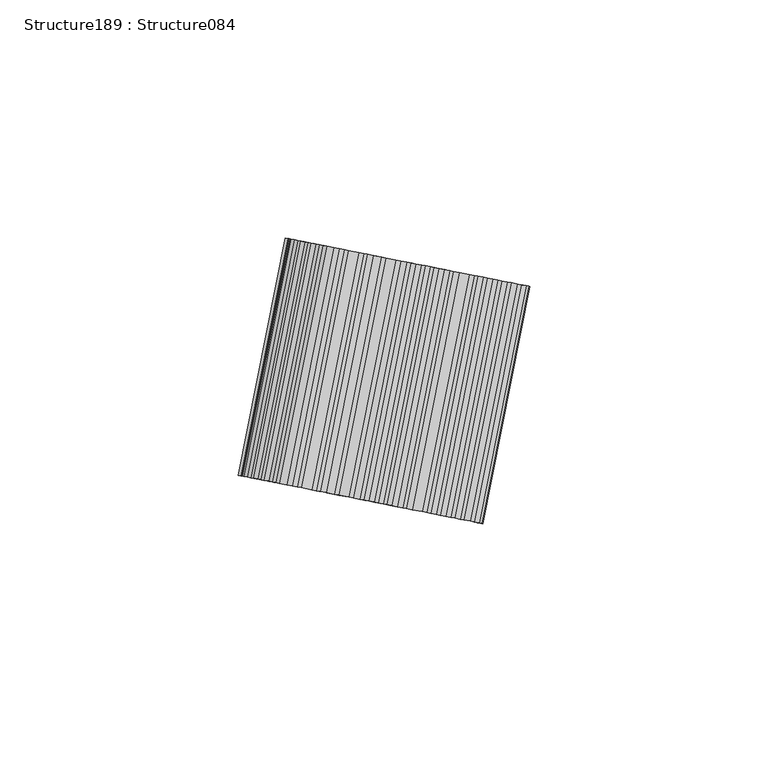
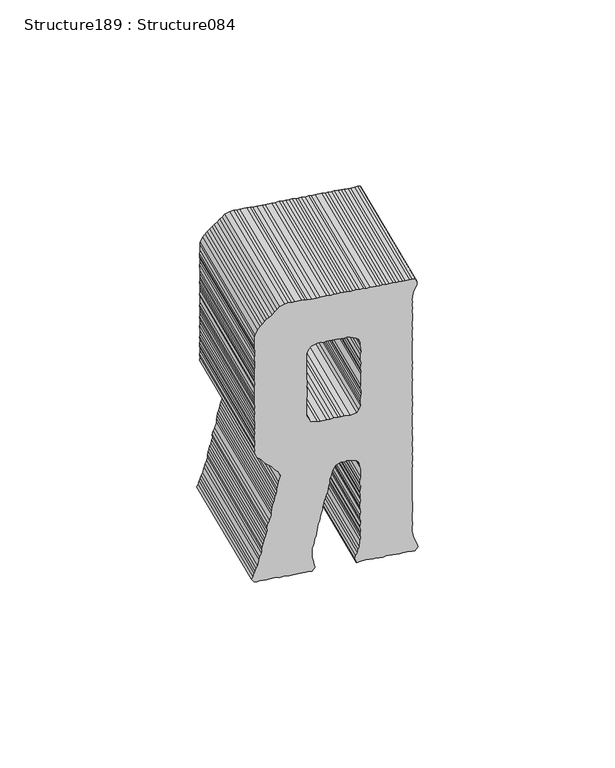
"""IFC4 building model written with IfcOpenShell, lengths in millimetres: proxy geometry, Structure189 : Structure084."""

from ifc_helpers import new_model, si_unit, frame, origin, place, context, project, spatial, polyline, outline, extrude, source, transform, mapped, element, save


def structure189_structure084_a6cd63ed(model_context):
    return source(origin(), model_context, "Body", "SweptSolid", [
        extrude(outline(polyline([(0.7877723, 0.0), (1.9464015, -0.1991228), (2.8602744, -0.225849), (4.1191818, -0.5725383), (5.014805, -0.7264607), (5.8881786, -1.0119464), (7.2131992, -0.9739456), (7.9618749, -1.2329462), (10.1385127, -1.6070246), (11.3090794, -1.6778664), (12.311293, -1.9804401), (13.2111243, -2.1350857), (14.2117928, -2.4424483), (15.4109212, -2.3828117), (16.5195828, -2.8390667), (17.4342994, -2.8608834), (18.6150357, -2.933473), (20.3591199, -3.4989322), (21.6394332, -3.7189677), (22.5801144, -3.6149141), (23.6845679, -4.0704459), (24.6308598, -3.9673566), (25.7800208, -4.1648522), (26.5039924, -4.5549941), (27.5279624, -4.7309743), (28.8526323, -4.6929133), (29.8357525, -5.1275927), (30.776083, -5.0234788), (32.5416935, -6.2493551), (32.9031424, -7.2342724), (33.5574941, -8.0085018), (34.477038, -8.823614), (35.0861234, -9.8507291), (35.972525, -11.5876372), (36.8685591, -12.5290416), (37.5229108, -13.303271), (37.9287766, -14.029741), (39.5076035, -14.8278254), (41.6445256, -14.6683321), (42.9644943, -14.6345176), (43.9051754, -14.530464), (45.0599472, -14.7289238), (46.0220341, -14.4982164), (46.9627152, -14.3941628), (48.1392433, -14.4660291), (49.0957798, -14.2340066), (50.041228, -14.1358267), (51.0844997, -14.1847914), (52.1563332, -14.1032778), (53.4327891, -14.3226503), (55.3194114, -14.1154471), (56.4288566, -13.779371), (57.6236345, -13.7240411), (58.7537019, -14.0536423), (59.5858309, -13.7955458), (60.7623591, -13.8674121), (61.6189076, -13.4882341), (62.7924221, -13.5545279), (63.7358265, -13.4556357), (64.9285003, -13.3999442), (65.8244741, -13.5539269), (66.898061, -13.4727145), (68.1350915, -13.1589264), (69.328609, -13.0983255), (71.318233, -13.0438502), (72.1765349, -12.6649735), (73.2419139, -12.587405), (74.0793029, -12.3302124), (75.2758945, -12.2748331), (76.003044, -11.8734165), (76.8931166, -12.8137963), (76.8480367, -13.8638733), (76.5842472, -14.6110041), (76.5400111, -15.6561716), (76.3416115, -16.8105927), (76.0343091, -17.8109106), (75.7045271, -19.7298024), (75.8093424, -20.6702534), (75.3295446, -21.9117003), (75.2811608, -23.7435663), (74.9337097, -25.0027039), (74.4272846, -27.9494232), (74.4005969, -28.8672741), (73.987756, -29.7191213), (74.0707545, -30.7865166), (72.6138584, -31.5939579), (71.7839977, -31.0552851), (70.7821347, -30.7527716), (69.6713689, -30.2961549), (68.9473974, -29.906013), (66.901912, -29.5544745), (65.7471403, -29.3560146), (64.7624532, -29.718225), (63.8447229, -29.6908359), (62.6738055, -29.6199339), (61.6840006, -29.9762104), (60.4904228, -30.0371621), (59.445047, -29.9878357), (58.3961644, -29.9379067), (57.3516982, -29.8937911), (56.362244, -30.2501279), (55.1913266, -30.1792259), (54.145107, -30.1348089), (53.0523006, -30.3383574), (52.1175809, -30.4434355), (51.2156457, -30.2884283), (50.0229718, -30.3441199), (48.9553464, -30.4263568), (47.8617565, -30.6344641), (47.0534221, -30.7562085), (45.832477, -30.9427894), (44.914396, -30.91534), (43.7173718, -30.9753383), (42.7766906, -31.079392), (41.494624, -30.8590552), (40.6854459, -30.985709), (39.5926997, -31.1889068), (38.2679695, -31.2273185), (36.4472301, -31.8368424), (35.5455414, -33.2664481), (35.3262292, -34.5425532), (34.9408158, -35.2684206), (34.9738469, -36.5929481), (35.1774557, -38.4731762), (35.8364483, -39.2435098), (37.3094464, -39.8927126), (38.4142507, -40.3483048), (41.3574633, -40.8541273), (42.4292967, -40.7726135), (43.70961, -40.9926491), (44.6888727, -41.4266656), (45.7377553, -41.4765946), (46.525177, -41.4765343), (47.5244428, -41.783656), (48.8103669, -42.0046557), (49.6810775, -42.2846293), (50.8784525, -42.2246912), (51.9076827, -42.4015754), (52.649904, -42.6645212), (53.6552737, -42.9676373), (54.9802942, -42.9296365), (56.0035629, -43.1054961), (56.8555307, -43.5176357), (57.7515045, -43.6716184), (58.9488796, -43.6116803), (60.0554372, -44.0675738), (61.0990597, -44.1165988), (61.869492, -44.2490058), (63.0007539, -44.5737579), (63.9372269, -44.468981), (66.2885299, -44.6124122), (67.125919, -44.3552198), (68.4493124, -44.3266872), (69.3028472, -43.9419368), (70.5019756, -43.8823), (71.6935756, -44.6185287), (71.3461245, -45.8776663), (70.9132807, -46.8564085), (70.759298, -47.7523823), (70.7307966, -48.6702824), (70.6639602, -49.846953), (70.3566579, -50.8472709), (70.3341179, -51.7661955), (70.1575351, -52.7936724), (69.7472914, -53.6409116), (69.69625, -54.689964), (69.3228948, -56.8623937), (69.2778149, -57.9124707), (68.992269, -58.786195), (68.6181303, -60.9631834), (68.5955903, -61.8821081), (68.4416077, -62.7780818), (67.1345464, -63.4762479), (66.0458878, -62.8930979), (65.1969939, -62.4861801), (64.1318451, -61.7767379), (63.4057694, -61.3862343), (61.4454907, -60.5179), (60.4218712, -60.3419801), (58.3267691, -60.2476341), (57.4807627, -59.8365192), (56.1757452, -59.7476251), (55.2985141, -59.4614765), (54.2305381, -59.5436531), (51.2834681, -59.0371677), (50.3063094, -58.6035128), (49.28269, -58.4275929), (47.9738151, -58.3380358), (46.0598327, -58.0090975), (45.0553067, -57.7010719), (44.0334407, -57.5254533), (42.9872211, -57.4810364), (39.0186357, -56.7989926), (37.9732599, -56.7496663), (36.9678903, -56.4465501), (35.6637165, -56.3527466), (34.6422011, -56.1771882), (33.8931746, -55.9181274), (32.8499028, -55.8691626), (31.5636281, -55.6481026), (30.5617652, -55.3455891), (29.6714021, -55.1925707), (28.7480611, -55.1642173), (27.5989002, -54.9667218), (26.7434256, -54.5539796), (25.5695604, -54.4876254), (24.5262885, -54.4386606), (23.4214843, -53.9830685), (22.6245944, -53.9815015), (21.6235752, -53.6740786), (20.3206618, -53.5855461), (19.2756365, -53.53628), (18.5509637, -53.1460175), (17.268897, -52.9256807), (16.4593683, -53.0522743), (15.300739, -52.8531514), (14.4321325, -52.5735395), (13.3871074, -52.5242734), (12.1225891, -52.1766198), (11.3803678, -51.9136741), (10.2086067, -51.8476815), (8.0263581, -51.4726388), (7.2362735, -51.4671869), (6.1085182, -51.1430375), (5.2354954, -50.8576121), (4.0800223, -50.6590317), (3.1400425, -50.7632059), (2.0122874, -50.4390565), (1.0892969, -50.4107634), (-0.1431529, -49.933234), (-1.1706297, -49.7566511), (-2.2147453, -49.7125958), (-2.9573172, -49.4495898), (-4.0087969, -49.4042689), (-5.0080628, -49.0971473), (-6.2887267, -48.8770515), (-7.1035156, -49.0027411), (-8.3620724, -48.656112), (-9.1102552, -48.3921417), (-10.1314198, -48.2166437), (-11.1997466, -48.29876), (-12.2051163, -47.9956439), (-13.4854295, -47.7756083), (-14.2776182, -47.7697949), (-16.3227529, -47.4183167), (-17.4331681, -46.9617603), (-18.4993908, -47.0442382), (-19.6267952, -46.7201491), (-20.6781325, -46.6697982), (-21.5523499, -46.3892219), (-23.7729936, -46.2733003), (-24.8401259, -46.3505675), (-25.6975181, -46.734655), (-26.7864672, -46.9388664), (-27.9612419, -46.8673015), (-28.903386, -46.1836924), (-28.8523447, -45.1346399), (-28.6983018, -44.2383154), (-28.3526042, -42.9788764), (-28.220378, -42.2094962), (-28.1483637, -41.0384089), (-27.8679957, -40.1591014), (-27.8177379, -39.1146076), (-27.6201821, -37.965096), (-27.3406578, -37.0906979), (-27.2677998, -35.9147012), (-27.010032, -35.1668965), (-26.9597742, -34.1224029), (-26.6073919, -32.072008), (-26.2616943, -30.8125691), (-26.3826552, -29.9996759), (-25.9319123, -28.8936772), (-25.9875436, -27.7006527), (-25.6832549, -26.6947624), (-25.4254871, -25.9469578), (-25.5028748, -24.8805269), (-25.2212466, -24.0064903), (-25.1513363, -22.8350415), (-24.8470476, -21.8291512), (-24.8207105, -20.9112402), (-24.3473674, -19.6737385), (-24.2963261, -18.624686), (-23.8191857, -16.6004256), (-23.6434466, -15.5778582), (-23.3571774, -13.9121535), (-23.1370214, -12.6311389), (-23.1311203, -11.8447418), (-23.0821829, -10.7953277), (-22.707984, -8.6179885), (-22.4263557, -7.743952), (-22.3782019, -6.6990967), (-21.9266152, -5.5881886), (-21.1449177, -4.1383221), (-20.1224106, -3.5266396), (-19.3473977, -2.8677292), (-18.3143703, -2.2578546), (-17.5002006, -1.3395928), (-16.8785896, -0.7897057), (-16.003649, -0.2783015), (-15.0749656, 0.4848928), (-14.3537777, 0.8873339), (-13.1940143, 1.480482), (-11.3979792, 1.9588644), (-10.4794051, 1.9363847), (-8.428309, 1.583882), (-7.1300967, 1.491103), (-6.3554563, 1.3579727), (-5.3765442, 0.9240165), (-4.3546782, 0.7483979), (-3.2867022, 0.8305746), (-1.0232687, 0.1758597), (0.0, 0.0), (0.7877723, 0.0)]), holes=[polyline([(18.9318372, -31.7250019), (19.2826525, -30.471497), (19.2842194, -29.674607), (19.5035317, -28.3985018), (19.9610799, -27.2886183), (20.0100172, -26.2392042), (20.4892615, -24.2153054), (20.3840956, -23.2747941), (20.4678464, -21.3085648), (19.6312408, -20.7734262), (18.3769139, -19.6354193), (17.4595343, -19.6080905), (16.1792211, -19.388055), (15.4301946, -19.1289941), (14.2771763, -18.9308356), (13.3629527, -18.9040492), (12.3417881, -18.7285511), (11.0337568, -18.6340846), (8.9865181, -18.2822448), (7.9811484, -17.9791286), (7.0630675, -17.9516793), (6.1670937, -17.7976966), (5.0614456, -17.3470139), (4.1654718, -17.1930312), (2.9889437, -17.1211649), (2.0926191, -16.967122), (1.0925096, -16.6649099), (-0.0840186, -16.5930436), (-0.9582359, -16.3124674), (-2.1130076, -16.1140075), (-3.0310886, -16.0865581), (-3.8996951, -15.8069462), (-5.5492761, -16.1852202), (-6.4511511, -16.8176346), (-7.5496121, -18.6044208), (-7.7253512, -19.6269882), (-7.6009438, -20.4408347), (-8.0334371, -21.4196372), (-8.5841586, -24.6241024), (-8.6784224, -25.9267529), (-8.6799072, -26.7189635), (-9.1123403, -27.6974153), (-9.0314457, -28.7644489), (-8.7006845, -30.671584), (-8.3169861, -31.524938), (-6.8689006, -32.3001919), (-5.9732774, -32.4541143), (-3.7094934, -33.1088896), (-2.7730203, -33.0041127), (-0.5967332, -33.3781309), (0.1279397, -33.7683934), (1.3044679, -33.8402597), (2.2230419, -33.8627393), (3.4554917, -34.3402688), (4.2455764, -34.3457206), (8.2162658, -35.028126), (9.3915337, -35.0947212), (10.2435015, -35.5068607), (11.272381, -35.6836847), (12.4436491, -35.754647), (13.3625738, -35.7771868), (14.3896999, -35.9537094), (15.6435555, -36.304585), (17.0346893, -35.8818941), (18.0463108, -35.3986734), (18.8829602, -33.5618376), (18.9318372, -31.7250019)])]), frame((-3137.0208819, 235091.0468772, 464.6145124), z_axis=(0.1946622229639412, 0.9808703374813293, 0.0), x_axis=(-0.1661373711927794, 0.0329714017826368, -0.9855512470478847)), (0.0, 0.0, 1.0), 50.8),
    ])


if __name__ == "__main__":
    model = new_model("IFC4")
    model_context = context("Model", 3, world=origin())
    ifc_project = project(units=[si_unit("LENGTHUNIT", "METRE", prefix="MILLI")], contexts=[model_context])
    site = spatial("IfcSite", under=ifc_project)
    building = spatial("IfcBuilding", under=site)
    placement = place(None, origin())
    structure189_structure084_shape = structure189_structure084_a6cd63ed(model_context)
    element("IfcBuildingElementProxy", 1, Name="Structure189 : Structure084", ObjectType="Structure189 : Structure084", at=placement, inside=building, context=model_context, shape_type="MappedRepresentation", body=[
        mapped(structure189_structure084_shape, transform((0.0, 0.0, 0.0), x_axis=(1.0, 0.0, 0.0), y_axis=(0.0, 1.0, 0.0), z_axis=(0.0, 0.0, 1.0))),
    ])
    save(model, "model.ifc")

# Revit data of these elements
# Type "Structure189 : Structure084"
#   NameOverride = "Structure084"
# Element 1 (IfcBuildingElementProxy, "Structure189 : Structure084")
#   Materials on its faces: "BRUSHED ALUMINUM LETTERING"
# Materials
#   "BRUSHED ALUMINUM LETTERING": class "Unassigned", colour RGB 169 181 186, transparency 0, Cost = 0
